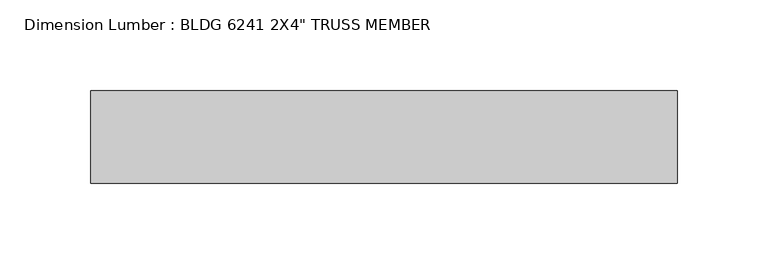
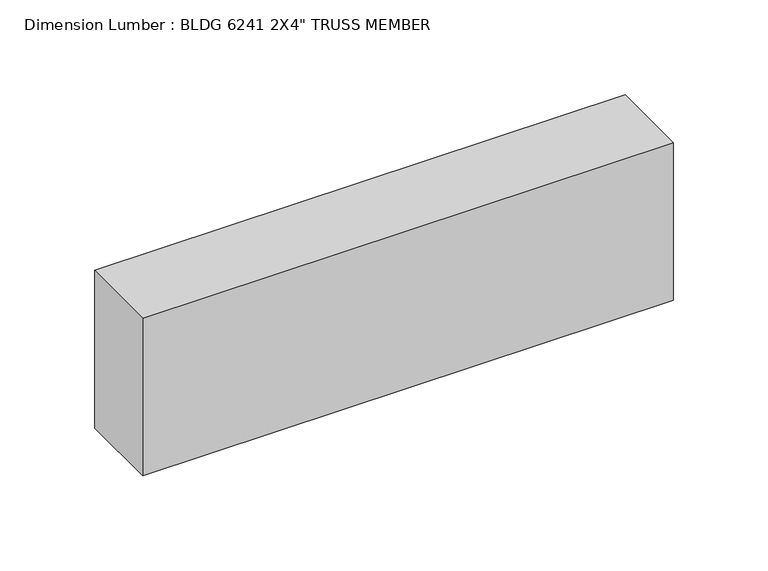
"""IFC4 building model written with IfcOpenShell, lengths in millimetres: beam geometry."""

from ifc_helpers import new_model, si_unit, frame, origin, place, context, project, spatial, polyline, outline, extrude, source, transform, mapped, element, save


def beam_8933aaf6(model_context):
    return source(origin(), model_context, "Body", "SweptSolid", [
        extrude(outline(polyline([(161.5124332, 25.4), (161.5124332, -25.4), (-161.5124332, -25.4), (-161.5124332, 25.4), (161.5124332, 25.4)])), frame((0.0, 0.0, -50.8), z_axis=(0.0, 0.0, 1.0), x_axis=(1.0, 0.0, 0.0)), (0.0, 0.0, 1.0), 101.6),
    ])


if __name__ == "__main__":
    model = new_model("IFC4")
    model_context = context("Model", 3, world=origin())
    ifc_project = project(units=[si_unit("LENGTHUNIT", "METRE", prefix="MILLI")], contexts=[model_context])
    site = spatial("IfcSite", under=ifc_project)
    building = spatial("IfcBuilding", under=site)
    placement = place(None, origin())
    beam_shape = beam_8933aaf6(model_context)
    element("IfcBeam", 1, ObjectType="Dimension Lumber : BLDG 6241 2X4\" TRUSS MEMBER", at=placement, inside=building, context=model_context, shape_type="MappedRepresentation", body=[
        mapped(beam_shape, transform((0.0, 0.0, 0.0), x_axis=(1.0, 0.0, 0.0), y_axis=(0.0, 1.0, 0.0), z_axis=(0.0, 0.0, 1.0))),
    ])
    save(model, "model.ifc")

# Revit data of these elements
# Type "Dimension Lumber : BLDG 6241 2X4\" TRUSS MEMBER"
#   Assembly Code = "B10"
#   A = 0.273472 SF
#   Length [instance default] = 5' - 0"
#   b = 0' - 2"
#   d = 0' - 4"
#   Structural Material [instance default] = Softwood, Lumber
# Element 1 (IfcBeam, "Dimension Lumber : BLDG 6241 2X4\" TRUSS MEMBER")
#   Materials on its faces: "Softwood, Lumber"
# Materials
#   "Softwood, Lumber": class "Wood", colour RGB 223 192 134, transparency 0, Description = "Pinus Echinata", Cost = 0
